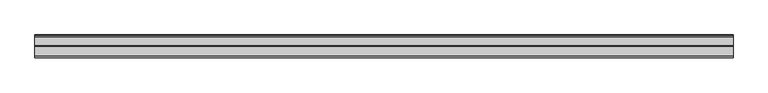
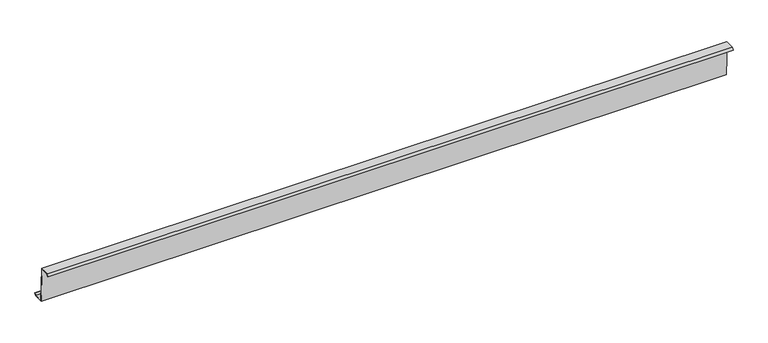
"""IFC4 building model written with IfcOpenShell, lengths in millimetres: proxy geometry, Generic Models 7:Generic Models 1:8:Generic Models 1:8 : Generic Models 7:Generic Models 1:337419:10 : Generic Models 7:Generic Models 1:8:Generic Models 1:8 : Generic Models 7:Generic Models 1:337419:315935."""

from ifc_helpers import new_model, si_unit, frame, origin, place, context, project, spatial, polyline, outline, extrude, source, transform, mapped, element, save


def generic_models_f5744a84(model_context):
    return source(origin(), model_context, "Body", "SweptSolid", [
        extrude(outline(polyline([(-563778.2601994, 8961.8878195), (-563713.427391, 8964.5891865), (-563702.9688875, 8713.5851025), (-563642.2061335, 8716.1168839), (-563631.3698368, 8730.1809633), (-563629.1691731, 8728.4853639), (-563640.7961408, 8713.3950981), (-563705.6289492, 8710.6937311), (-563716.0874527, 8961.6978151), (-563776.8198905, 8959.1672968), (-563787.6680911, 8945.0877677), (-563789.8871671, 8946.7975537), (-563778.2601994, 8961.8878195)])), frame((591306.0367242, 0.0, 0.0), z_axis=(1.0, 0.0, 0.0), x_axis=(0.0, 1.0, 0.0)), (0.0, 0.0, 1.0), 4876.8),
    ])


if __name__ == "__main__":
    model = new_model("IFC4")
    model_context = context("Model", 3, world=origin())
    ifc_project = project(units=[si_unit("LENGTHUNIT", "METRE", prefix="MILLI")], contexts=[model_context])
    site = spatial("IfcSite", under=ifc_project)
    building = spatial("IfcBuilding", under=site)
    placement = place(None, origin())
    generic_models_shape = generic_models_f5744a84(model_context)
    element("IfcBuildingElementProxy", 1, Name="Generic Models 7:Generic Models 1:8:Generic Models 1:8 : Generic Models 7:Generic Models 1:337419:10 : Generic Models 7:Generic Models 1:8:Generic Models 1:8 : Generic Models 7:Generic Models 1:337419:315935", ObjectType="Generic Models 7:Generic Models 1:8:Generic Models 1:8 : Generic Models 7:Generic Models 1:337419:10 : Generic Models 7:Generic Models 1:8:Generic Models 1:8 : Generic Models 7:Generic Models 1:337419:315935", at=placement, inside=building, context=model_context, shape_type="MappedRepresentation", body=[
        mapped(generic_models_shape, transform((0.0, 0.0, 0.0), x_axis=(1.0, 0.0, 0.0), y_axis=(0.0, 1.0, 0.0), z_axis=(0.0, 0.0, 1.0))),
    ])
    save(model, "model.ifc")

# Revit data of these elements
# Type "Generic Models 7:Generic Models 1:8:Generic Models 1:8 : Generic Models 7:Generic Models 1:337419:10 : Generic Models 7:Generic Models 1:8:Generic Models 1:8 : Generic Models 7:Generic Models 1:337419:315935"
#   NameOverride = "Generic Models 7:Generic Models 1:8:Generic Models 1:8 : Generic Models 7:Generic Models 1:337419:315935"
#   ObjectTypeOverride = "Generic Models 1:8 : Generic Models 7:Generic Models 1:337419"
#   Reference = "Generic Models 1"
#   Tag = "315935"
# Element 1 (IfcBuildingElementProxy, "Generic Models 7:Generic Models 1:8:Generic Models 1:8 : Generic Models 7:Generic Models 1:337419:10 : Generic Models 7:Generic Models 1:8:Generic Models 1:8 : Generic Models 7:Generic Models 1:337419:315935")
#   Materials on its faces: "ZEE' PURLIN (SEE STRUCT. DWGS)"
# Materials
#   "ZEE' PURLIN (SEE STRUCT. DWGS)": class "Unassigned", colour RGB 210 209 208, transparency 0, Cost = 0
